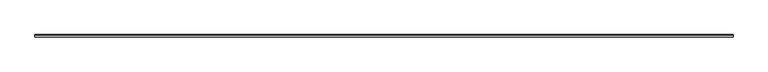
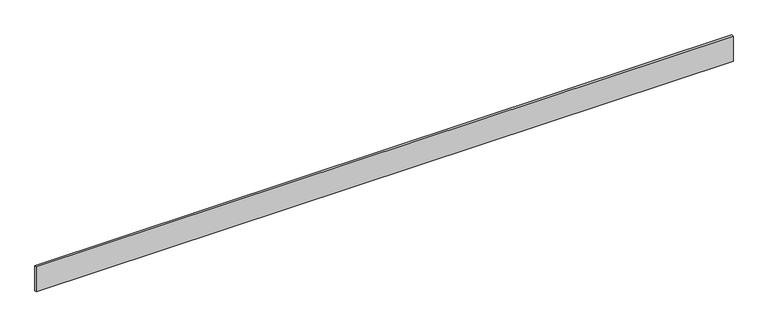
"""IFC4 building model written with IfcOpenShell, lengths in millimetres: proxy geometry, Generic Models 7:Generic Models 1:8:Generic Models 1:8 : Generic Models 7:Generic Models 1:337419:11 : Generic Models 7:Generic Models 1:8:Generic Models 1:8 : Generic Models 7:Generic Models 1:337419:315935."""

from ifc_helpers import new_model, si_unit, frame, origin, place, context, project, spatial, polyline, outline, extrude, source, transform, mapped, element, save


def generic_models_c73ddf9a(model_context):
    return source(origin(), model_context, "Body", "SweptSolid", [
        extrude(outline(polyline([(-568227.4010637, 8760.5211374), (-568226.5898179, 8759.7098917), (-568226.5898179, 8576.3711374), (-568242.4648179, 8576.3711374), (-568242.4648179, 8760.5211374), (-568227.4010637, 8760.5211374)])), frame((591306.0367242, 0.0, 0.0), z_axis=(1.0, 0.0, 0.0), x_axis=(0.0, 1.0, 0.0)), (0.0, 0.0, 1.0), 4876.8),
    ])


if __name__ == "__main__":
    model = new_model("IFC4")
    model_context = context("Model", 3, world=origin())
    ifc_project = project(units=[si_unit("LENGTHUNIT", "METRE", prefix="MILLI")], contexts=[model_context])
    site = spatial("IfcSite", under=ifc_project)
    building = spatial("IfcBuilding", under=site)
    placement = place(None, origin())
    generic_models_shape = generic_models_c73ddf9a(model_context)
    element("IfcBuildingElementProxy", 1, Name="Generic Models 7:Generic Models 1:8:Generic Models 1:8 : Generic Models 7:Generic Models 1:337419:11 : Generic Models 7:Generic Models 1:8:Generic Models 1:8 : Generic Models 7:Generic Models 1:337419:315935", ObjectType="Generic Models 7:Generic Models 1:8:Generic Models 1:8 : Generic Models 7:Generic Models 1:337419:11 : Generic Models 7:Generic Models 1:8:Generic Models 1:8 : Generic Models 7:Generic Models 1:337419:315935", at=placement, inside=building, context=model_context, shape_type="MappedRepresentation", body=[
        mapped(generic_models_shape, transform((0.0, 0.0, 0.0), x_axis=(1.0, 0.0, 0.0), y_axis=(0.0, 1.0, 0.0), z_axis=(0.0, 0.0, 1.0))),
    ])
    save(model, "model.ifc")

# Revit data of these elements
# Type "Generic Models 7:Generic Models 1:8:Generic Models 1:8 : Generic Models 7:Generic Models 1:337419:11 : Generic Models 7:Generic Models 1:8:Generic Models 1:8 : Generic Models 7:Generic Models 1:337419:315935"
#   NameOverride = "Generic Models 7:Generic Models 1:8:Generic Models 1:8 : Generic Models 7:Generic Models 1:337419:315935"
#   ObjectTypeOverride = "Generic Models 1:8 : Generic Models 7:Generic Models 1:337419"
#   Reference = "Generic Models 1"
#   Tag = "315935"
# Element 1 (IfcBuildingElementProxy, "Generic Models 7:Generic Models 1:8:Generic Models 1:8 : Generic Models 7:Generic Models 1:337419:11 : Generic Models 7:Generic Models 1:8:Generic Models 1:8 : Generic Models 7:Generic Models 1:337419:315935")
#   Materials on its faces: "ENGINEERED WOOD TRIM (LP SMARTSIDE)"
# Materials
#   "ENGINEERED WOOD TRIM (LP SMARTSIDE)": class "Wood", colour RGB 108 80 40, transparency 0, Description = "Pinus Echinata", Cost = 0
